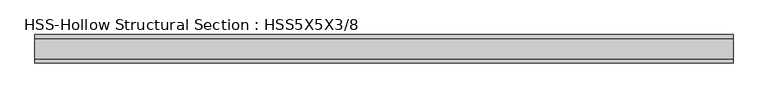
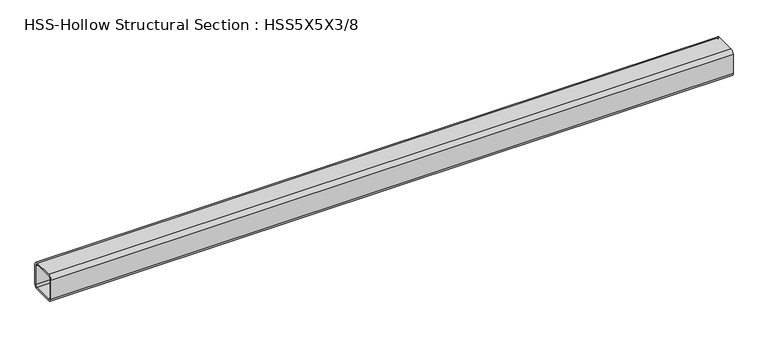
"""IFC4 building model written with IfcOpenShell, lengths in millimetres: member geometry, HSS-Hollow Structural Section : HSS5X5X3/8."""

import ifcopenshell
import ifcopenshell.guid

model = None  # the IFC model being written
_history = None  # IfcOwnerHistory: only IFC2X3 demands one
_inside = {}  # id of a spatial element -> (the spatial element, [elements in it])
_under = {}  # id of a project, library or spatial element -> (it, [spatial elements below it])
_declared = {}  # id of a project -> (the project, [libraries it declares])
_typed = {}  # id of a type object -> (the type object, [elements of that type])
_made_of = {}  # id of a material, layer set ... -> (it, [elements and type objects made of it])


def new_model(schema):
    """Start an empty IFC model of exactly this schema.

    Asked for "IFC4X3", IfcOpenShell would pick the latest addendum, in which some entities
    have other attributes; the version numbers below select the first issue.
    IFC2X3 requires an IfcOwnerHistory on every rooted entity: one is made here for all.
    """
    global model, _history
    if schema == "IFC4X3":
        model = ifcopenshell.file(schema_version=(4, 3, 0, 0))
    else:
        model = ifcopenshell.file(schema=schema)
    _inside.clear()
    _under.clear()
    _declared.clear()
    _typed.clear()
    _made_of.clear()
    _history = None
    if model.schema == "IFC2X3":
        org = make("IfcOrganization", Name="unknown")
        user = make(
            "IfcPersonAndOrganization",
            ThePerson=make("IfcPerson", FamilyName="unknown"),
            TheOrganization=org,
        )
        app = make(
            "IfcApplication",
            ApplicationDeveloper=org,
            Version="unknown",
            ApplicationFullName="unknown",
            ApplicationIdentifier="unknown",
        )
        _history = make(
            "IfcOwnerHistory",
            OwningUser=user,
            OwningApplication=app,
            ChangeAction="ADDED",
            CreationDate=0,
        )
    return model


def make(cls, **values):
    """One entity of the class cls with the attributes given. An attribute that is None is left unset."""
    return model.create_entity(
        cls, **{name: value for name, value in values.items() if value is not None}
    )


def rooted(cls, **values):
    """An entity with a GlobalId (a new one), such as an element, a storey or a relation."""
    return make(cls, GlobalId=ifcopenshell.guid.new(), OwnerHistory=_history, **values)


def si_unit(unit_type, name, prefix=None):
    """IfcSIUnit, for example si_unit("LENGTHUNIT", "METRE", prefix="MILLI")."""
    return make("IfcSIUnit", UnitType=unit_type, Prefix=prefix, Name=name)


def assignment(units):
    """IfcUnitAssignment: the units of a project."""
    return None if units is None else make("IfcUnitAssignment", Units=units)


def point(xyz):
    """IfcCartesianPoint."""
    return None if xyz is None else make("IfcCartesianPoint", Coordinates=xyz)


def direction(xyz):
    """IfcDirection."""
    return None if xyz is None else make("IfcDirection", DirectionRatios=xyz)


def frame(location, z_axis=None, x_axis=None):
    """IfcAxis2Placement3D, a coordinate frame: its origin and axes. An axis left out is left unset."""
    return make(
        "IfcAxis2Placement3D",
        Location=point(location),
        Axis=direction(z_axis),
        RefDirection=direction(x_axis),
    )


def frame_2d(location, x_axis=None):
    """IfcAxis2Placement2D, a coordinate frame in the plane: its origin and x axis."""
    return make(
        "IfcAxis2Placement2D", Location=point(location), RefDirection=direction(x_axis)
    )


def origin():
    """The frame at (0, 0, 0) with its axes left unset."""
    return frame((0.0, 0.0, 0.0))


def place(relative_to, where):
    """IfcLocalPlacement: puts the frame where relative to a parent placement (None: the world)."""
    return make(
        "IfcLocalPlacement", PlacementRelTo=relative_to, RelativePlacement=where
    )


def context(
    kind, dimensions, precision=None, world=None, true_north=None, identifier=None
):
    """IfcGeometricRepresentationContext, for example the 3D "Model" context."""
    return make(
        "IfcGeometricRepresentationContext",
        ContextIdentifier=identifier,
        ContextType=kind,
        CoordinateSpaceDimension=dimensions,
        Precision=precision,
        WorldCoordinateSystem=world,
        TrueNorth=true_north,
    )


def project(units=None, contexts=None):
    """IfcProject with its units and contexts."""
    return rooted(
        "IfcProject",
        Name="project",
        RepresentationContexts=contexts,
        UnitsInContext=assignment(units),
    )


def spatial(cls, under=None, at=None, **own):
    """A site, building, storey or space (cls), placed at a placement, below another one or the project."""
    s = rooted(cls, ObjectPlacement=at, **own)
    if under is not None:
        _under.setdefault(under.id(), (under, []))[1].append(s)
    return s


def polyline(points):
    """IfcPolyline through the points."""
    return make("IfcPolyline", Points=[point(p) for p in points])


def circle_curve(where, radius):
    """IfcCircle in the frame where."""
    return make("IfcCircle", Position=where, Radius=radius)


def trimmed(basis, trim1, trim2, sense, master):
    """IfcTrimmedCurve: the piece of a basis curve between two trims."""
    return make(
        "IfcTrimmedCurve",
        BasisCurve=basis,
        Trim1=trim1,
        Trim2=trim2,
        SenseAgreement=sense,
        MasterRepresentation=master,
    )


def segment(curve, same_sense, transition):
    """IfcCompositeCurveSegment."""
    return make(
        "IfcCompositeCurveSegment",
        Transition=transition,
        SameSense=same_sense,
        ParentCurve=curve,
    )


def composite_curve(segments, self_intersect=None):
    """IfcCompositeCurve: segments joined end to end."""
    return make("IfcCompositeCurve", Segments=segments, SelfIntersect=self_intersect)


def outline(outer, holes=None, kind="AREA"):
    """IfcArbitraryClosedProfileDef: a profile drawn as a closed curve; with holes, ...WithVoids."""
    if holes is None:
        return make("IfcArbitraryClosedProfileDef", ProfileType=kind, OuterCurve=outer)
    return make(
        "IfcArbitraryProfileDefWithVoids",
        ProfileType=kind,
        OuterCurve=outer,
        InnerCurves=holes,
    )


def extrude(swept, where, along, depth):
    """IfcExtrudedAreaSolid: the profile swept, set in the frame where, extruded along a direction by depth."""
    return make(
        "IfcExtrudedAreaSolid",
        SweptArea=swept,
        Position=where,
        ExtrudedDirection=direction(along),
        Depth=depth,
    )


def shape(context_of_items, identifier, shape_type, items):
    """IfcShapeRepresentation: the items that make up one representation, for example the "Body"."""
    return make(
        "IfcShapeRepresentation",
        ContextOfItems=context_of_items,
        RepresentationIdentifier=identifier,
        RepresentationType=shape_type,
        Items=items,
    )


def source(mapping_origin, context_of_items, identifier, shape_type, items):
    """IfcRepresentationMap: a shape defined once, which mapped items show again and again."""
    return make(
        "IfcRepresentationMap",
        MappingOrigin=mapping_origin,
        MappedRepresentation=shape(context_of_items, identifier, shape_type, items),
    )


def transform(
    local_origin,
    x_axis=None,
    y_axis=None,
    z_axis=None,
    scale=None,
    scale2=None,
    scale3=None,
    uniform=True,
):
    """IfcCartesianTransformationOperator3D, or its non-uniform kind. x_axis, y_axis, z_axis: its Axis1, 2, 3."""
    if uniform:
        return make(
            "IfcCartesianTransformationOperator3D",
            Axis1=direction(x_axis),
            Axis2=direction(y_axis),
            LocalOrigin=point(local_origin),
            Scale=scale,
            Axis3=direction(z_axis),
        )
    return make(
        "IfcCartesianTransformationOperator3DnonUniform",
        Axis1=direction(x_axis),
        Axis2=direction(y_axis),
        LocalOrigin=point(local_origin),
        Scale=scale,
        Axis3=direction(z_axis),
        Scale2=scale2,
        Scale3=scale3,
    )


def mapped(mapping_source, mapping_target):
    """IfcMappedItem: shows the shape of a source again, moved by a transform."""
    return make(
        "IfcMappedItem", MappingSource=mapping_source, MappingTarget=mapping_target
    )


def made_of(thing, what):
    """Note that an element or type object is made of a material, layer set ...; save() writes the relation."""
    if what is not None:
        _made_of.setdefault(what.id(), (what, []))[1].append(thing)
    return thing


def element(
    cls,
    number,
    at=None,
    inside=None,
    cuts=None,
    type_object=None,
    material=None,
    context=None,
    identifier="Body",
    shape_type=None,
    held_by="IfcProductDefinitionShape",
    body=None,
    shapes=None,
    **own,
):
    """One element of the class cls, such as IfcWall. Its Tag is "e" and its number.

    at: its placement. inside: the storey or other place that contains it. cuts: it is an
    opening in that element (IfcRelVoidsElement). A single representation is given by context,
    identifier, shape_type and body (its items); several are given by shapes. held_by: the class
    of the entity that holds the representations. save() writes the other relations.
    """
    e = rooted(cls, Tag="e%d" % number, ObjectPlacement=at, **own)
    if body is not None:
        shapes = [shape(context, identifier, shape_type, body)]
    if shapes is not None:
        e.Representation = make(held_by, Representations=shapes)
    if inside is not None:
        _inside.setdefault(inside.id(), (inside, []))[1].append(e)
    if cuts is not None:
        rooted(
            "IfcRelVoidsElement", RelatingBuildingElement=cuts, RelatedOpeningElement=e
        )
    if type_object is not None:
        _typed.setdefault(type_object.id(), (type_object, []))[1].append(e)
    return made_of(e, material)


def aggregate(whole, parts):
    """IfcRelAggregates: a whole, such as a stair, and the parts it consists of."""
    return rooted("IfcRelAggregates", RelatingObject=whole, RelatedObjects=parts)


def save(model, path):
    """Write the relations noted so far, then the file.

    IfcRelAggregates (storeys below a building ...), IfcRelContainedInSpatialStructure (elements
    in a storey), IfcRelDefinesByType, IfcRelAssociatesMaterial and IfcRelDeclares: one each for
    every whole, place, type object, material and project.
    """
    for whole, parts in _under.values():
        aggregate(whole, parts)
    for where, things in _inside.values():
        rooted(
            "IfcRelContainedInSpatialStructure",
            RelatedElements=things,
            RelatingStructure=where,
        )
    for kind, things in _typed.values():
        rooted("IfcRelDefinesByType", RelatedObjects=things, RelatingType=kind)
    for what, things in _made_of.values():
        rooted("IfcRelAssociatesMaterial", RelatedObjects=things, RelatingMaterial=what)
    for by, libraries in _declared.values():
        rooted("IfcRelDeclares", RelatingContext=by, RelatedDefinitions=libraries)
    model.write(path)


def hss_hollow_structural_section_hss5x5x3_8_66eacc37(model_context):
    return source(origin(), model_context, "Body", "SweptSolid", [
        extrude(outline(composite_curve([segment(polyline([(63.5, 45.7708), (63.5, -45.7708)]), True, "CONTINUOUS"), segment(trimmed(circle_curve(frame_2d((45.7708, -45.7708)), 17.7292), [point((63.5, -45.7708))], [point((45.7708, -63.5))], False, "CARTESIAN"), True, "CONTINUOUS"), segment(polyline([(45.7708, -63.5), (-45.7708, -63.5)]), True, "CONTINUOUS"), segment(trimmed(circle_curve(frame_2d((-45.7708, -45.7708)), 17.7292), [point((-45.7708, -63.5))], [point((-63.5, -45.7708))], False, "CARTESIAN"), True, "CONTINUOUS"), segment(polyline([(-63.5, -45.7708), (-63.5, 45.7708)]), True, "CONTINUOUS"), segment(trimmed(circle_curve(frame_2d((-45.7708, 45.7708)), 17.7292), [point((-63.5, 45.7708))], [point((-45.7708, 63.5))], False, "CARTESIAN"), True, "CONTINUOUS"), segment(polyline([(-45.7708, 63.5), (45.7708, 63.5)]), True, "CONTINUOUS"), segment(trimmed(circle_curve(frame_2d((45.7708, 45.7708)), 17.7292), [point((45.7708, 63.5))], [point((63.5, 45.7708))], False, "CARTESIAN"), True, "CONTINUOUS")], self_intersect=False), holes=[composite_curve([segment(trimmed(circle_curve(frame_2d((-45.7708, 45.7708)), 8.8646), [point((-45.7708, 54.6354))], [point((-54.6354, 45.7708))], True, "CARTESIAN"), True, "CONTINUOUS"), segment(polyline([(-54.6354, 45.7708), (-54.6354, -45.7708)]), True, "CONTINUOUS"), segment(trimmed(circle_curve(frame_2d((-45.7708, -45.7708)), 8.8646), [point((-54.6354, -45.7708))], [point((-45.7708, -54.6354))], True, "CARTESIAN"), True, "CONTINUOUS"), segment(polyline([(-45.7708, -54.6354), (45.7708, -54.6354)]), True, "CONTINUOUS"), segment(trimmed(circle_curve(frame_2d((45.7708, -45.7708)), 8.8646), [point((45.7708, -54.6354))], [point((54.6354, -45.7708))], True, "CARTESIAN"), True, "CONTINUOUS"), segment(polyline([(54.6354, -45.7708), (54.6354, 45.7708)]), True, "CONTINUOUS"), segment(trimmed(circle_curve(frame_2d((45.7708, 45.7708)), 8.8646), [point((54.6354, 45.7708))], [point((45.7708, 54.6354))], True, "CARTESIAN"), True, "CONTINUOUS"), segment(polyline([(45.7708, 54.6354), (-45.7708, 54.6354)]), True, "CONTINUOUS")], self_intersect=False)]), frame((-1563.4187975, 0.0, 0.0), z_axis=(1.0, 0.0, 0.0), x_axis=(0.0, 1.0, 0.0)), (0.0, 0.0, 1.0), 3126.8375951),
    ])


if __name__ == "__main__":
    model = new_model("IFC4")
    model_context = context("Model", 3, world=origin())
    ifc_project = project(units=[si_unit("LENGTHUNIT", "METRE", prefix="MILLI")], contexts=[model_context])
    site = spatial("IfcSite", under=ifc_project)
    building = spatial("IfcBuilding", under=site)
    placement = place(None, origin())
    hss_hollow_structural_section_hss5x5x3_8_shape = hss_hollow_structural_section_hss5x5x3_8_66eacc37(model_context)
    element("IfcMember", 1, ObjectType="HSS-Hollow Structural Section : HSS5X5X3/8", at=placement, inside=building, context=model_context, shape_type="MappedRepresentation", body=[
        mapped(hss_hollow_structural_section_hss5x5x3_8_shape, transform((0.0, 0.0, 0.0), x_axis=(1.0, 0.0, 0.0), y_axis=(0.0, 1.0, 0.0), z_axis=(0.0, 0.0, 1.0))),
    ])
    save(model, "model.ifc")

# Revit data of these elements
# Type "HSS-Hollow Structural Section : HSS5X5X3/8"
#   Assembly Code = "B10"
#   Shape = "Square"
#   W = 22.3
#   Ht = 0' - 5"
#   Length [instance default] = 5' - 0"
#   b = 0' - 5"
#   kr = 0' - 0.698"
#   t = 0' - 0.349"
#   A = 0.0429167 SF
#   Structural Material [instance default] = Steel ASTM A500, Grade B, Rectangular and Square
# Element 1 (IfcMember, "HSS-Hollow Structural Section : HSS5X5X3/8")
#   Materials on its faces: "Steel ASTM A500, Grade B, Rectangular and Square"
# Materials
#   "Steel ASTM A500, Grade B, Rectangular and Square": class "Metal", colour RGB 199 199 199, transparency 0, Description = "Carbon steel", Cost = 0
